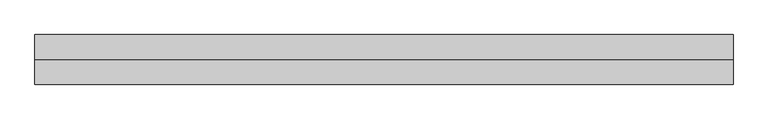
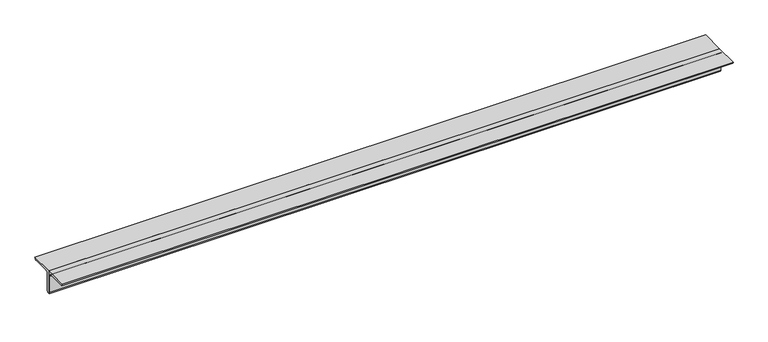
"""IFC4 building model written with IfcOpenShell, lengths in millimetres: member geometry, 0123_Steel Framing_2Ls-KSD3502 : H_SB_AR_S03_2Ls-130x130x12_HBR4."""

from ifc_helpers import new_model, si_unit, point, frame, frame_2d, origin, place, context, project, spatial, polyline, circle_curve, trimmed, segment, composite_curve, outline, extrude, source, transform, mapped, element, save


def member_ff9c955f(model_context):
    return source(origin(), model_context, "Body", "SweptSolid", [
        extrude(outline(composite_curve([segment(polyline([(0.0, 36.4), (130.0, 36.4)]), True, "CONTINUOUS"), segment(trimmed(circle_curve(frame_2d((118.0, 36.4)), 12.0), [point((130.0, 36.4))], [point((118.0, 24.4))], False, "CARTESIAN"), True, "CONTINUOUS"), segment(polyline([(118.0, 24.4), (24.0, 24.4)]), True, "CONTINUOUS"), segment(trimmed(circle_curve(frame_2d((24.0, 12.4)), 12.0), [point((24.0, 24.4))], [point((12.0, 12.4))], True, "CARTESIAN"), True, "CONTINUOUS"), segment(polyline([(12.0, 12.4), (12.0, -81.6)]), True, "CONTINUOUS"), segment(trimmed(circle_curve(frame_2d((0.0, -81.6)), 12.0), [point((12.0, -81.6))], [point((0.0, -93.6))], False, "CARTESIAN"), True, "CONTINUOUS"), segment(polyline([(0.0, -93.6), (0.0, 36.4)]), True, "CONTINUOUS")], self_intersect=False)), frame((-1720.2330278, 0.0, 0.0), z_axis=(1.0, 0.0, 0.0), x_axis=(0.0, 1.0, 0.0)), (0.0, 0.0, 1.0), 3660.0954461),
        extrude(outline(composite_curve([segment(polyline([(0.0, 36.4), (0.0, -93.6)]), True, "CONTINUOUS"), segment(trimmed(circle_curve(frame_2d((0.0, -81.6)), 12.0), [point((0.0, -93.6))], [point((-12.0, -81.6))], False, "CARTESIAN"), True, "CONTINUOUS"), segment(polyline([(-12.0, -81.6), (-12.0, 12.4)]), True, "CONTINUOUS"), segment(trimmed(circle_curve(frame_2d((-24.0, 12.4)), 12.0), [point((-12.0, 12.4))], [point((-24.0, 24.4))], True, "CARTESIAN"), True, "CONTINUOUS"), segment(polyline([(-24.0, 24.4), (-118.0, 24.4)]), True, "CONTINUOUS"), segment(trimmed(circle_curve(frame_2d((-118.0, 36.4)), 12.0), [point((-118.0, 24.4))], [point((-130.0, 36.4))], False, "CARTESIAN"), True, "CONTINUOUS"), segment(polyline([(-130.0, 36.4), (0.0, 36.4)]), True, "CONTINUOUS")], self_intersect=False)), frame((-1720.2330278, 0.0, 0.0), z_axis=(1.0, 0.0, 0.0), x_axis=(0.0, 1.0, 0.0)), (0.0, 0.0, 1.0), 3660.0954461),
    ])


if __name__ == "__main__":
    model = new_model("IFC4")
    model_context = context("Model", 3, world=origin())
    ifc_project = project(units=[si_unit("LENGTHUNIT", "METRE", prefix="MILLI")], contexts=[model_context])
    site = spatial("IfcSite", under=ifc_project)
    building = spatial("IfcBuilding", under=site)
    placement = place(None, origin())
    member_shape = member_ff9c955f(model_context)
    element("IfcMember", 1, ObjectType="0123_Steel Framing_2Ls-KSD3502 : H_SB_AR_S03_2Ls-130x130x12_HBR4", at=placement, inside=building, context=model_context, shape_type="MappedRepresentation", body=[
        mapped(member_shape, transform((0.0, 0.0, 0.0), x_axis=(1.0, 0.0, 0.0), y_axis=(0.0, 1.0, 0.0), z_axis=(0.0, 0.0, 1.0))),
    ])
    save(model, "model.ifc")

# Revit data of these elements
# Type "0123_Steel Framing_2Ls-KSD3502 : H_SB_AR_S03_2Ls-130x130x12_HBR4"
#   Assembly Code = "B10"
#   Legs = "SLBB"
#   W = 8.97
#   Perimeter = 1.04 m²/m
#   Nominal Weight = 46.80 kgf/m
#   Length [instance default] = 1000 mm
#   Space = 0 mm
#   b = 130 mm
#   d = 130 mm
#   t = 12 mm
#   y = 36.4 mm
#   A = 0.005952 m²
#   Structural Material [instance default] = Steel ASTM A36
# Element 1 (IfcMember, "0123_Steel Framing_2Ls-KSD3502 : H_SB_AR_S03_2Ls-130x130x12_HBR4")
#   Structural Material = Steel, 45-345
#   Materials on its faces: "Steel, 45-345"
# Materials
#   "Steel ASTM A36": class "Metal", colour RGB 199 199 199, transparency 0, Description = "Structural steel, ASTM A36 Grade B, mill finish", Cost = 0
#   "Steel, 45-345": class "Metal", colour RGB 189 187 185, transparency 0, Description = "Steel 345 MPa", Cost = 0
